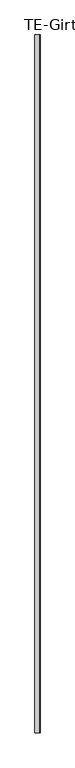
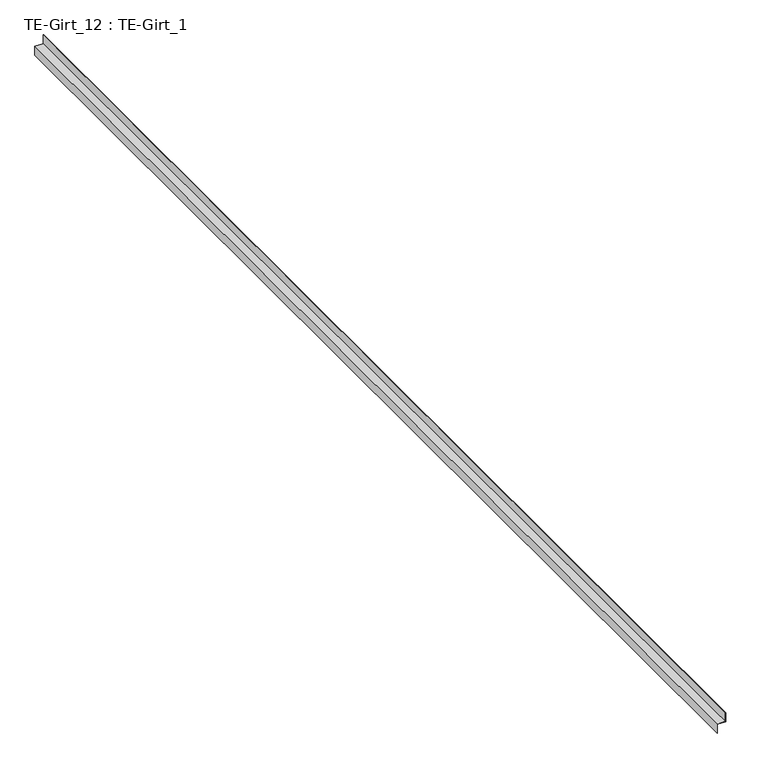
"""IFC4 building model written with IfcOpenShell, lengths in millimetres: proxy geometry, TE-Girt_12 : TE-Girt_1."""

from ifc_helpers import new_model, si_unit, frame, origin, place, context, project, spatial, polyline, outline, extrude, source, transform, mapped, element, save


def te_girt_12_te_girt_1_6a4ee48b(model_context):
    return source(origin(), model_context, "Body", "SweptSolid", [
        extrude(outline(polyline([(2374.9, 590353.5827614), (2413.0, 590353.5827614), (2413.0, 590352.6897927), (2375.7929688, 590352.6897927), (2375.7929688, 590318.6434739), (2337.6929688, 590318.6434739), (2337.6929688, 590319.5364427), (2374.9, 590319.5364427), (2374.9, 590353.5827614)])), frame((0.0, -536417.5913841, 0.0), z_axis=(0.0, 1.0, 0.0), x_axis=(0.0, 0.0, 1.0)), (0.0, 0.0, 1.0), 4777.4820312),
    ])


if __name__ == "__main__":
    model = new_model("IFC4")
    model_context = context("Model", 3, world=origin())
    ifc_project = project(units=[si_unit("LENGTHUNIT", "METRE", prefix="MILLI")], contexts=[model_context])
    site = spatial("IfcSite", under=ifc_project)
    building = spatial("IfcBuilding", under=site)
    placement = place(None, origin())
    te_girt_12_te_girt_1_shape = te_girt_12_te_girt_1_6a4ee48b(model_context)
    element("IfcBuildingElementProxy", 1, Name="TE-Girt_12 : TE-Girt_1", ObjectType="TE-Girt_12 : TE-Girt_1", at=placement, inside=building, context=model_context, shape_type="MappedRepresentation", body=[
        mapped(te_girt_12_te_girt_1_shape, transform((0.0, 0.0, 0.0), x_axis=(1.0, 0.0, 0.0), y_axis=(0.0, 1.0, 0.0), z_axis=(0.0, 0.0, 1.0))),
    ])
    save(model, "model.ifc")

# Revit data of these elements
# Element 1 (IfcBuildingElementProxy, "TE-Girt_12 : TE-Girt_1")
#   Materials on its faces: "Z-FURRING, COLD-FORMED GALV."
# Materials
#   "Z-FURRING, COLD-FORMED GALV.": class "Generic", colour RGB 143 142 141, transparency 0, Cost = 0
